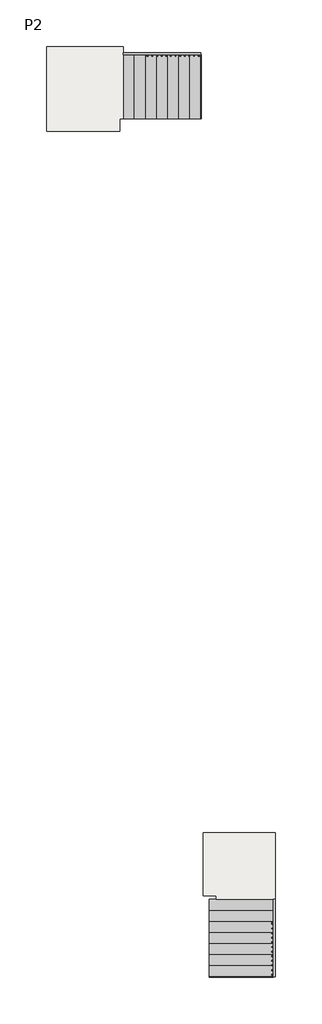
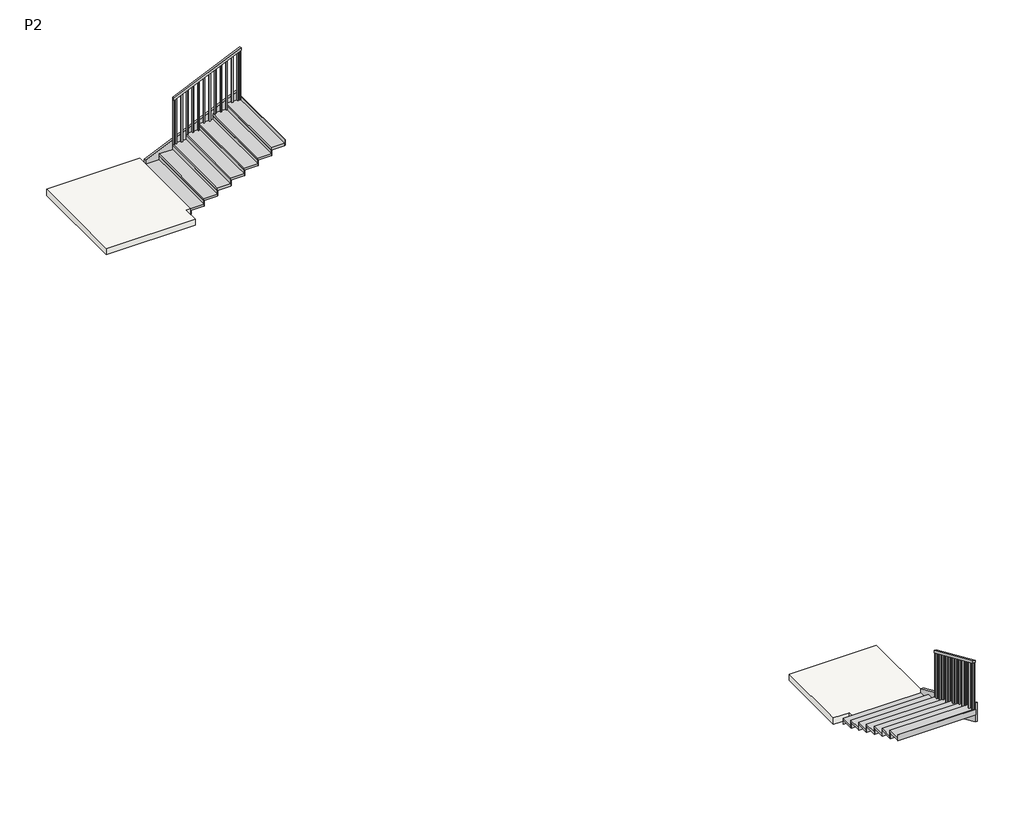
# One storey: 2 members, 2 railings, 2 slabs, 2 stair flights.
"""IFC4 building model written with IfcOpenShell, lengths in millimetres."""

import ifcopenshell
import ifcopenshell.guid

model = None  # the IFC model being written
_history = None  # IfcOwnerHistory: only IFC2X3 demands one
_inside = {}  # id of a spatial element -> (the spatial element, [elements in it])
_under = {}  # id of a project, library or spatial element -> (it, [spatial elements below it])
_declared = {}  # id of a project -> (the project, [libraries it declares])
_typed = {}  # id of a type object -> (the type object, [elements of that type])
_made_of = {}  # id of a material, layer set ... -> (it, [elements and type objects made of it])


def new_model(schema):
    """Start an empty IFC model of exactly this schema.

    Asked for "IFC4X3", IfcOpenShell would pick the latest addendum, in which some entities
    have other attributes; the version numbers below select the first issue.
    IFC2X3 requires an IfcOwnerHistory on every rooted entity: one is made here for all.
    """
    global model, _history
    if schema == "IFC4X3":
        model = ifcopenshell.file(schema_version=(4, 3, 0, 0))
    else:
        model = ifcopenshell.file(schema=schema)
    _inside.clear()
    _under.clear()
    _declared.clear()
    _typed.clear()
    _made_of.clear()
    _history = None
    if model.schema == "IFC2X3":
        org = make("IfcOrganization", Name="unknown")
        user = make(
            "IfcPersonAndOrganization",
            ThePerson=make("IfcPerson", FamilyName="unknown"),
            TheOrganization=org,
        )
        app = make(
            "IfcApplication",
            ApplicationDeveloper=org,
            Version="unknown",
            ApplicationFullName="unknown",
            ApplicationIdentifier="unknown",
        )
        _history = make(
            "IfcOwnerHistory",
            OwningUser=user,
            OwningApplication=app,
            ChangeAction="ADDED",
            CreationDate=0,
        )
    return model


def make(cls, **values):
    """One entity of the class cls with the attributes given. An attribute that is None is left unset."""
    return model.create_entity(
        cls, **{name: value for name, value in values.items() if value is not None}
    )


def rooted(cls, **values):
    """An entity with a GlobalId (a new one), such as an element, a storey or a relation."""
    return make(cls, GlobalId=ifcopenshell.guid.new(), OwnerHistory=_history, **values)


def si_unit(unit_type, name, prefix=None):
    """IfcSIUnit, for example si_unit("LENGTHUNIT", "METRE", prefix="MILLI")."""
    return make("IfcSIUnit", UnitType=unit_type, Prefix=prefix, Name=name)


def assignment(units):
    """IfcUnitAssignment: the units of a project."""
    return None if units is None else make("IfcUnitAssignment", Units=units)


def point(xyz):
    """IfcCartesianPoint."""
    return None if xyz is None else make("IfcCartesianPoint", Coordinates=xyz)


def direction(xyz):
    """IfcDirection."""
    return None if xyz is None else make("IfcDirection", DirectionRatios=xyz)


def frame(location, z_axis=None, x_axis=None):
    """IfcAxis2Placement3D, a coordinate frame: its origin and axes. An axis left out is left unset."""
    return make(
        "IfcAxis2Placement3D",
        Location=point(location),
        Axis=direction(z_axis),
        RefDirection=direction(x_axis),
    )


def origin():
    """The frame at (0, 0, 0) with its axes left unset."""
    return frame((0.0, 0.0, 0.0))


def place(relative_to, where):
    """IfcLocalPlacement: puts the frame where relative to a parent placement (None: the world)."""
    return make(
        "IfcLocalPlacement", PlacementRelTo=relative_to, RelativePlacement=where
    )


def context(
    kind, dimensions, precision=None, world=None, true_north=None, identifier=None
):
    """IfcGeometricRepresentationContext, for example the 3D "Model" context."""
    return make(
        "IfcGeometricRepresentationContext",
        ContextIdentifier=identifier,
        ContextType=kind,
        CoordinateSpaceDimension=dimensions,
        Precision=precision,
        WorldCoordinateSystem=world,
        TrueNorth=true_north,
    )


def project(units=None, contexts=None):
    """IfcProject with its units and contexts."""
    return rooted(
        "IfcProject",
        Name="project",
        RepresentationContexts=contexts,
        UnitsInContext=assignment(units),
    )


def spatial(cls, under=None, at=None, **own):
    """A site, building, storey or space (cls), placed at a placement, below another one or the project."""
    s = rooted(cls, ObjectPlacement=at, **own)
    if under is not None:
        _under.setdefault(under.id(), (under, []))[1].append(s)
    return s


def polyline(points):
    """IfcPolyline through the points."""
    return make("IfcPolyline", Points=[point(p) for p in points])


def outline(outer, holes=None, kind="AREA"):
    """IfcArbitraryClosedProfileDef: a profile drawn as a closed curve; with holes, ...WithVoids."""
    if holes is None:
        return make("IfcArbitraryClosedProfileDef", ProfileType=kind, OuterCurve=outer)
    return make(
        "IfcArbitraryProfileDefWithVoids",
        ProfileType=kind,
        OuterCurve=outer,
        InnerCurves=holes,
    )


def extrude(swept, where, along, depth):
    """IfcExtrudedAreaSolid: the profile swept, set in the frame where, extruded along a direction by depth."""
    return make(
        "IfcExtrudedAreaSolid",
        SweptArea=swept,
        Position=where,
        ExtrudedDirection=direction(along),
        Depth=depth,
    )


def shape(context_of_items, identifier, shape_type, items):
    """IfcShapeRepresentation: the items that make up one representation, for example the "Body"."""
    return make(
        "IfcShapeRepresentation",
        ContextOfItems=context_of_items,
        RepresentationIdentifier=identifier,
        RepresentationType=shape_type,
        Items=items,
    )


def source(mapping_origin, context_of_items, identifier, shape_type, items):
    """IfcRepresentationMap: a shape defined once, which mapped items show again and again."""
    return make(
        "IfcRepresentationMap",
        MappingOrigin=mapping_origin,
        MappedRepresentation=shape(context_of_items, identifier, shape_type, items),
    )


def transform(
    local_origin,
    x_axis=None,
    y_axis=None,
    z_axis=None,
    scale=None,
    scale2=None,
    scale3=None,
    uniform=True,
):
    """IfcCartesianTransformationOperator3D, or its non-uniform kind. x_axis, y_axis, z_axis: its Axis1, 2, 3."""
    if uniform:
        return make(
            "IfcCartesianTransformationOperator3D",
            Axis1=direction(x_axis),
            Axis2=direction(y_axis),
            LocalOrigin=point(local_origin),
            Scale=scale,
            Axis3=direction(z_axis),
        )
    return make(
        "IfcCartesianTransformationOperator3DnonUniform",
        Axis1=direction(x_axis),
        Axis2=direction(y_axis),
        LocalOrigin=point(local_origin),
        Scale=scale,
        Axis3=direction(z_axis),
        Scale2=scale2,
        Scale3=scale3,
    )


def mapped(mapping_source, mapping_target):
    """IfcMappedItem: shows the shape of a source again, moved by a transform."""
    return make(
        "IfcMappedItem", MappingSource=mapping_source, MappingTarget=mapping_target
    )


def made_of(thing, what):
    """Note that an element or type object is made of a material, layer set ...; save() writes the relation."""
    if what is not None:
        _made_of.setdefault(what.id(), (what, []))[1].append(thing)
    return thing


def element(
    cls,
    number,
    at=None,
    inside=None,
    cuts=None,
    type_object=None,
    material=None,
    context=None,
    identifier="Body",
    shape_type=None,
    held_by="IfcProductDefinitionShape",
    body=None,
    shapes=None,
    **own,
):
    """One element of the class cls, such as IfcWall. Its Tag is "e" and its number.

    at: its placement. inside: the storey or other place that contains it. cuts: it is an
    opening in that element (IfcRelVoidsElement). A single representation is given by context,
    identifier, shape_type and body (its items); several are given by shapes. held_by: the class
    of the entity that holds the representations. save() writes the other relations.
    """
    e = rooted(cls, Tag="e%d" % number, ObjectPlacement=at, **own)
    if body is not None:
        shapes = [shape(context, identifier, shape_type, body)]
    if shapes is not None:
        e.Representation = make(held_by, Representations=shapes)
    if inside is not None:
        _inside.setdefault(inside.id(), (inside, []))[1].append(e)
    if cuts is not None:
        rooted(
            "IfcRelVoidsElement", RelatingBuildingElement=cuts, RelatedOpeningElement=e
        )
    if type_object is not None:
        _typed.setdefault(type_object.id(), (type_object, []))[1].append(e)
    return made_of(e, material)


def aggregate(whole, parts):
    """IfcRelAggregates: a whole, such as a stair, and the parts it consists of."""
    return rooted("IfcRelAggregates", RelatingObject=whole, RelatedObjects=parts)


def save(model, path):
    """Write the relations noted so far, then the file.

    IfcRelAggregates (storeys below a building ...), IfcRelContainedInSpatialStructure (elements
    in a storey), IfcRelDefinesByType, IfcRelAssociatesMaterial and IfcRelDeclares: one each for
    every whole, place, type object, material and project.
    """
    for whole, parts in _under.values():
        aggregate(whole, parts)
    for where, things in _inside.values():
        rooted(
            "IfcRelContainedInSpatialStructure",
            RelatedElements=things,
            RelatingStructure=where,
        )
    for kind, things in _typed.values():
        rooted("IfcRelDefinesByType", RelatedObjects=things, RelatingType=kind)
    for what, things in _made_of.values():
        rooted("IfcRelAssociatesMaterial", RelatedObjects=things, RelatingMaterial=what)
    for by, libraries in _declared.values():
        rooted("IfcRelDeclares", RelatingContext=by, RelatedDefinitions=libraries)
    model.write(path)


def stair_flight_50mm_tread_13mm_riser_cadf6dc6(model_context):
    return source(origin(), model_context, "Body", "SweptSolid", [
        extrude(outline(polyline([(-15531.918089, 15530.6768963), (-15544.418089, 15530.6768963), (-15544.418089, 17260.6768963), (-15531.918089, 17260.6768963), (-15531.918089, 15530.6768963)])), frame((0.0, 0.0, -1066.6666667), z_axis=(0.0, 0.0, 1.0), x_axis=(1.0, 0.0, 0.0)), (0.0, 0.0, 1.0), 83.3333333),
        extrude(outline(polyline([(-15244.418089, 17260.6768963), (-15244.418089, 15530.6768963), (-15544.418089, 15530.6768963), (-15544.418089, 17260.6768963), (-15244.418089, 17260.6768963)])), frame((0.0, 0.0, -983.3333333), z_axis=(0.0, 0.0, 1.0), x_axis=(1.0, 0.0, 0.0)), (0.0, 0.0, 1.0), 50.0),
        extrude(outline(polyline([(-15231.918089, 15530.6768963), (-15244.418089, 15530.6768963), (-15244.418089, 17260.6768963), (-15231.918089, 17260.6768963), (-15231.918089, 15530.6768963)])), frame((0.0, 0.0, -983.3333333), z_axis=(0.0, 0.0, 1.0), x_axis=(1.0, 0.0, 0.0)), (0.0, 0.0, 1.0), 133.3333333),
        extrude(outline(polyline([(-14944.418089, 17260.6768963), (-14944.418089, 15530.6768963), (-15244.418089, 15530.6768963), (-15244.418089, 17260.6768963), (-14944.418089, 17260.6768963)])), frame((0.0, 0.0, -850.0), z_axis=(0.0, 0.0, 1.0), x_axis=(1.0, 0.0, 0.0)), (0.0, 0.0, 1.0), 50.0),
        extrude(outline(polyline([(-14931.918089, 15530.6768963), (-14944.418089, 15530.6768963), (-14944.418089, 17260.6768963), (-14931.918089, 17260.6768963), (-14931.918089, 15530.6768963)])), frame((0.0, 0.0, -850.0), z_axis=(0.0, 0.0, 1.0), x_axis=(1.0, 0.0, 0.0)), (0.0, 0.0, 1.0), 133.3333333),
        extrude(outline(polyline([(-14644.418089, 17260.6768963), (-14644.418089, 15530.6768963), (-14944.418089, 15530.6768963), (-14944.418089, 17260.6768963), (-14644.418089, 17260.6768963)])), frame((0.0, 0.0, -716.6666667), z_axis=(0.0, 0.0, 1.0), x_axis=(1.0, 0.0, 0.0)), (0.0, 0.0, 1.0), 50.0),
        extrude(outline(polyline([(-14631.918089, 15530.6768963), (-14644.418089, 15530.6768963), (-14644.418089, 17260.6768963), (-14631.918089, 17260.6768963), (-14631.918089, 15530.6768963)])), frame((0.0, 0.0, -716.6666667), z_axis=(0.0, 0.0, 1.0), x_axis=(1.0, 0.0, 0.0)), (0.0, 0.0, 1.0), 133.3333333),
        extrude(outline(polyline([(-14344.418089, 17260.6768963), (-14344.418089, 15530.6768963), (-14644.418089, 15530.6768963), (-14644.418089, 17260.6768963), (-14344.418089, 17260.6768963)])), frame((0.0, 0.0, -583.3333333), z_axis=(0.0, 0.0, 1.0), x_axis=(1.0, 0.0, 0.0)), (0.0, 0.0, 1.0), 50.0),
        extrude(outline(polyline([(-14331.918089, 15530.6768963), (-14344.418089, 15530.6768963), (-14344.418089, 17260.6768963), (-14331.918089, 17260.6768963), (-14331.918089, 15530.6768963)])), frame((0.0, 0.0, -583.3333333), z_axis=(0.0, 0.0, 1.0), x_axis=(1.0, 0.0, 0.0)), (0.0, 0.0, 1.0), 133.3333333),
        extrude(outline(polyline([(-14044.418089, 17260.6768963), (-14044.418089, 15530.6768963), (-14344.418089, 15530.6768963), (-14344.418089, 17260.6768963), (-14044.418089, 17260.6768963)])), frame((0.0, 0.0, -450.0), z_axis=(0.0, 0.0, 1.0), x_axis=(1.0, 0.0, 0.0)), (0.0, 0.0, 1.0), 50.0),
        extrude(outline(polyline([(-14031.918089, 15530.6768963), (-14044.418089, 15530.6768963), (-14044.418089, 17260.6768963), (-14031.918089, 17260.6768963), (-14031.918089, 15530.6768963)])), frame((0.0, 0.0, -450.0), z_axis=(0.0, 0.0, 1.0), x_axis=(1.0, 0.0, 0.0)), (0.0, 0.0, 1.0), 133.3333333),
        extrude(outline(polyline([(-13744.418089, 17260.6768963), (-13744.418089, 15530.6768963), (-14044.418089, 15530.6768963), (-14044.418089, 17260.6768963), (-13744.418089, 17260.6768963)])), frame((0.0, 0.0, -316.6666667), z_axis=(0.0, 0.0, 1.0), x_axis=(1.0, 0.0, 0.0)), (0.0, 0.0, 1.0), 50.0),
        extrude(outline(polyline([(-13731.918089, 15530.6768963), (-13744.418089, 15530.6768963), (-13744.418089, 17260.6768963), (-13731.918089, 17260.6768963), (-13731.918089, 15530.6768963)])), frame((0.0, 0.0, -316.6666667), z_axis=(0.0, 0.0, 1.0), x_axis=(1.0, 0.0, 0.0)), (0.0, 0.0, 1.0), 133.3333333),
        extrude(outline(polyline([(-13431.918089, 15530.6768963), (-13444.418089, 15530.6768963), (-13444.418089, 17260.6768963), (-13431.918089, 17260.6768963), (-13431.918089, 15530.6768963)])), frame((0.0, 0.0, -183.3333333), z_axis=(0.0, 0.0, 1.0), x_axis=(1.0, 0.0, 0.0)), (0.0, 0.0, 1.0), 133.3333333),
        extrude(outline(polyline([(-13444.418089, 17260.6768963), (-13444.418089, 15530.6768963), (-13744.418089, 15530.6768963), (-13744.418089, 17260.6768963), (-13444.418089, 17260.6768963)])), frame((0.0, 0.0, -183.3333333), z_axis=(0.0, 0.0, 1.0), x_axis=(1.0, 0.0, 0.0)), (0.0, 0.0, 1.0), 50.0),
    ])


def stair_flight_50mm_tread_13mm_riser_d40b31cd(model_context):
    return source(origin(), model_context, "Body", "SweptSolid", [
        extrude(outline(polyline([(-13215.2814495, -5630.5731037), (-13215.2814495, -5618.0731037), (-11485.2814495, -5618.0731037), (-11485.2814495, -5630.5731037), (-13215.2814495, -5630.5731037)])), frame((0.0, 0.0, -1066.6666667), z_axis=(0.0, 0.0, 1.0), x_axis=(1.0, 0.0, 0.0)), (0.0, 0.0, 1.0), 83.3333333),
        extrude(outline(polyline([(-11485.2814495, -5918.0731037), (-13215.2814495, -5918.0731037), (-13215.2814495, -5618.0731037), (-11485.2814495, -5618.0731037), (-11485.2814495, -5918.0731037)])), frame((0.0, 0.0, -983.3333333), z_axis=(0.0, 0.0, 1.0), x_axis=(1.0, 0.0, 0.0)), (0.0, 0.0, 1.0), 50.0),
        extrude(outline(polyline([(-13215.2814495, -5930.5731037), (-13215.2814495, -5918.0731037), (-11485.2814495, -5918.0731037), (-11485.2814495, -5930.5731037), (-13215.2814495, -5930.5731037)])), frame((0.0, 0.0, -983.3333333), z_axis=(0.0, 0.0, 1.0), x_axis=(1.0, 0.0, 0.0)), (0.0, 0.0, 1.0), 133.3333333),
        extrude(outline(polyline([(-11485.2814495, -6218.0731037), (-13215.2814495, -6218.0731037), (-13215.2814495, -5918.0731037), (-11485.2814495, -5918.0731037), (-11485.2814495, -6218.0731037)])), frame((0.0, 0.0, -850.0), z_axis=(0.0, 0.0, 1.0), x_axis=(1.0, 0.0, 0.0)), (0.0, 0.0, 1.0), 50.0),
        extrude(outline(polyline([(-13215.2814495, -6230.5731037), (-13215.2814495, -6218.0731037), (-11485.2814495, -6218.0731037), (-11485.2814495, -6230.5731037), (-13215.2814495, -6230.5731037)])), frame((0.0, 0.0, -850.0), z_axis=(0.0, 0.0, 1.0), x_axis=(1.0, 0.0, 0.0)), (0.0, 0.0, 1.0), 133.3333333),
        extrude(outline(polyline([(-11485.2814495, -6518.0731037), (-13215.2814495, -6518.0731037), (-13215.2814495, -6218.0731037), (-11485.2814495, -6218.0731037), (-11485.2814495, -6518.0731037)])), frame((0.0, 0.0, -716.6666667), z_axis=(0.0, 0.0, 1.0), x_axis=(1.0, 0.0, 0.0)), (0.0, 0.0, 1.0), 50.0),
        extrude(outline(polyline([(-13215.2814495, -6530.5731037), (-13215.2814495, -6518.0731037), (-11485.2814495, -6518.0731037), (-11485.2814495, -6530.5731037), (-13215.2814495, -6530.5731037)])), frame((0.0, 0.0, -716.6666667), z_axis=(0.0, 0.0, 1.0), x_axis=(1.0, 0.0, 0.0)), (0.0, 0.0, 1.0), 133.3333333),
        extrude(outline(polyline([(-11485.2814495, -6818.0731037), (-13215.2814495, -6818.0731037), (-13215.2814495, -6518.0731037), (-11485.2814495, -6518.0731037), (-11485.2814495, -6818.0731037)])), frame((0.0, 0.0, -583.3333333), z_axis=(0.0, 0.0, 1.0), x_axis=(1.0, 0.0, 0.0)), (0.0, 0.0, 1.0), 50.0),
        extrude(outline(polyline([(-13215.2814495, -6830.5731037), (-13215.2814495, -6818.0731037), (-11485.2814495, -6818.0731037), (-11485.2814495, -6830.5731037), (-13215.2814495, -6830.5731037)])), frame((0.0, 0.0, -583.3333333), z_axis=(0.0, 0.0, 1.0), x_axis=(1.0, 0.0, 0.0)), (0.0, 0.0, 1.0), 133.3333333),
        extrude(outline(polyline([(-11485.2814495, -7118.0731037), (-13215.2814495, -7118.0731037), (-13215.2814495, -6818.0731037), (-11485.2814495, -6818.0731037), (-11485.2814495, -7118.0731037)])), frame((0.0, 0.0, -450.0), z_axis=(0.0, 0.0, 1.0), x_axis=(1.0, 0.0, 0.0)), (0.0, 0.0, 1.0), 50.0),
        extrude(outline(polyline([(-13215.2814495, -7130.5731037), (-13215.2814495, -7118.0731037), (-11485.2814495, -7118.0731037), (-11485.2814495, -7130.5731037), (-13215.2814495, -7130.5731037)])), frame((0.0, 0.0, -450.0), z_axis=(0.0, 0.0, 1.0), x_axis=(1.0, 0.0, 0.0)), (0.0, 0.0, 1.0), 133.3333333),
        extrude(outline(polyline([(-11485.2814495, -7418.0731037), (-13215.2814495, -7418.0731037), (-13215.2814495, -7118.0731037), (-11485.2814495, -7118.0731037), (-11485.2814495, -7418.0731037)])), frame((0.0, 0.0, -316.6666667), z_axis=(0.0, 0.0, 1.0), x_axis=(1.0, 0.0, 0.0)), (0.0, 0.0, 1.0), 50.0),
        extrude(outline(polyline([(-13215.2814495, -7430.5731037), (-13215.2814495, -7418.0731037), (-11485.2814495, -7418.0731037), (-11485.2814495, -7430.5731037), (-13215.2814495, -7430.5731037)])), frame((0.0, 0.0, -316.6666667), z_axis=(0.0, 0.0, 1.0), x_axis=(1.0, 0.0, 0.0)), (0.0, 0.0, 1.0), 133.3333333),
        extrude(outline(polyline([(-13215.2814495, -7730.5731037), (-13215.2814495, -7718.0731037), (-11485.2814495, -7718.0731037), (-11485.2814495, -7730.5731037), (-13215.2814495, -7730.5731037)])), frame((0.0, 0.0, -183.3333333), z_axis=(0.0, 0.0, 1.0), x_axis=(1.0, 0.0, 0.0)), (0.0, 0.0, 1.0), 133.3333333),
        extrude(outline(polyline([(-11485.2814495, -7718.0731037), (-13215.2814495, -7718.0731037), (-13215.2814495, -7418.0731037), (-11485.2814495, -7418.0731037), (-11485.2814495, -7718.0731037)])), frame((0.0, 0.0, -183.3333333), z_axis=(0.0, 0.0, 1.0), x_axis=(1.0, 0.0, 0.0)), (0.0, 0.0, 1.0), 50.0),
    ])


model = new_model("IFC4")

# Units and contexts
model_context = context("Model", 3, world=origin())
ifc_project = project(units=[si_unit("LENGTHUNIT", "METRE", prefix="MILLI")], contexts=[model_context])

# Site, building, storey
site = spatial("IfcSite", under=ifc_project)
building = spatial("IfcBuilding", under=site)
storey = spatial("IfcBuildingStorey", under=building, Name="P2", Elevation=-1066.6666667)

# Members
placement = place(None, origin())
element("IfcMember", 1, ObjectType="Stringer - 50mm Width", at=placement, inside=storey, context=model_context, shape_type="SweptSolid", body=[
    extrude(outline(polyline([(-848.6428388, -15544.418089), (-1066.6666667, -15544.418089), (-1066.6666667, -15050.0859214), (-353.0365189, -13444.418089), (84.6904945, -13444.418089), (-848.6428388, -15544.418089)])), frame((0.0, 17260.6768963, 0.0), z_axis=(0.0, 1.0, 0.0), x_axis=(0.0, 0.0, 1.0)), (0.0, 0.0, 1.0), 50.0),
])
element("IfcMember", 2, ObjectType="Stringer - 50mm Width", at=placement, inside=storey, context=model_context, shape_type="SweptSolid", body=[
    extrude(outline(polyline([(-5618.0731037, -848.6428388), (-5618.0731037, -1066.6666667), (-6112.4052712, -1066.6666667), (-7718.0731037, -353.0365189), (-7718.0731037, 84.6904945), (-5618.0731037, -848.6428388)])), frame((-11485.2814495, 0.0, 0.0), z_axis=(1.0, 0.0, 0.0), x_axis=(0.0, 1.0, 0.0)), (0.0, 0.0, 1.0), 50.0),
])

# Railings
element("IfcRailing", 3, ObjectType="1100mm", at=placement, inside=storey, context=model_context, shape_type="SweptSolid", body=[
    extrude(outline(polyline([(433.3333333, -14944.418089), (378.6174567, -14944.418089), (1045.2841233, -13444.418089), (1100.0, -13444.418089), (433.3333333, -14944.418089)])), frame((0.0, 17210.2768963, 0.0), z_axis=(0.0, 1.0, 0.0), x_axis=(0.0, 0.0, 1.0)), (0.0, 0.0, 1.0), 50.0),
    extrude(outline(polyline([(-133.3333333, -13519.418089), (-133.3333333, -13494.418089), (1023.0619011, -13494.418089), (1011.95079, -13519.418089), (-133.3333333, -13519.418089)])), frame((0.0, 17222.7768963, 0.0), z_axis=(0.0, 1.0, 0.0), x_axis=(0.0, 0.0, 1.0)), (0.0, 0.0, 1.0), 25.0),
    extrude(outline(polyline([(-133.3333333, -13644.418089), (-133.3333333, -13619.418089), (967.5063455, -13619.418089), (956.3952344, -13644.418089), (-133.3333333, -13644.418089)])), frame((0.0, 17222.7768963, 0.0), z_axis=(0.0, 1.0, 0.0), x_axis=(0.0, 0.0, 1.0)), (0.0, 0.0, 1.0), 25.0),
    extrude(outline(polyline([(-266.6666667, -13769.418089), (-266.6666667, -13744.418089), (911.95079, -13744.418089), (900.8396789, -13769.418089), (-266.6666667, -13769.418089)])), frame((0.0, 17222.7768963, 0.0), z_axis=(0.0, 1.0, 0.0), x_axis=(0.0, 0.0, 1.0)), (0.0, 0.0, 1.0), 25.0),
    extrude(outline(polyline([(-266.6666667, -13894.418089), (-266.6666667, -13869.418089), (856.3952344, -13869.418089), (845.2841233, -13894.418089), (-266.6666667, -13894.418089)])), frame((0.0, 17222.7768963, 0.0), z_axis=(0.0, 1.0, 0.0), x_axis=(0.0, 0.0, 1.0)), (0.0, 0.0, 1.0), 25.0),
    extrude(outline(polyline([(-266.6666667, -14019.418089), (-266.6666667, -13994.418089), (800.8396789, -13994.418089), (789.7285678, -14019.418089), (-266.6666667, -14019.418089)])), frame((0.0, 17222.7768963, 0.0), z_axis=(0.0, 1.0, 0.0), x_axis=(0.0, 0.0, 1.0)), (0.0, 0.0, 1.0), 25.0),
    extrude(outline(polyline([(-400.0, -14144.418089), (-400.0, -14119.418089), (745.2841233, -14119.418089), (734.1730122, -14144.418089), (-400.0, -14144.418089)])), frame((0.0, 17222.7768963, 0.0), z_axis=(0.0, 1.0, 0.0), x_axis=(0.0, 0.0, 1.0)), (0.0, 0.0, 1.0), 25.0),
    extrude(outline(polyline([(-400.0, -14269.418089), (-400.0, -14244.418089), (689.7285678, -14244.418089), (678.6174567, -14269.418089), (-400.0, -14269.418089)])), frame((0.0, 17222.7768963, 0.0), z_axis=(0.0, 1.0, 0.0), x_axis=(0.0, 0.0, 1.0)), (0.0, 0.0, 1.0), 25.0),
    extrude(outline(polyline([(-533.3333333, -14394.418089), (-533.3333333, -14369.418089), (634.1730122, -14369.418089), (623.0619011, -14394.418089), (-533.3333333, -14394.418089)])), frame((0.0, 17222.7768963, 0.0), z_axis=(0.0, 1.0, 0.0), x_axis=(0.0, 0.0, 1.0)), (0.0, 0.0, 1.0), 25.0),
    extrude(outline(polyline([(-533.3333333, -14519.418089), (-533.3333333, -14494.418089), (578.6174567, -14494.418089), (567.5063455, -14519.418089), (-533.3333333, -14519.418089)])), frame((0.0, 17222.7768963, 0.0), z_axis=(0.0, 1.0, 0.0), x_axis=(0.0, 0.0, 1.0)), (0.0, 0.0, 1.0), 25.0),
    extrude(outline(polyline([(-533.3333333, -14644.418089), (-533.3333333, -14619.418089), (523.0619011, -14619.418089), (511.95079, -14644.418089), (-533.3333333, -14644.418089)])), frame((0.0, 17222.7768963, 0.0), z_axis=(0.0, 1.0, 0.0), x_axis=(0.0, 0.0, 1.0)), (0.0, 0.0, 1.0), 25.0),
    extrude(outline(polyline([(-666.6666667, -14769.418089), (-666.6666667, -14744.418089), (467.5063455, -14744.418089), (456.3952344, -14769.418089), (-666.6666667, -14769.418089)])), frame((0.0, 17222.7768963, 0.0), z_axis=(0.0, 1.0, 0.0), x_axis=(0.0, 0.0, 1.0)), (0.0, 0.0, 1.0), 25.0),
    extrude(outline(polyline([(-666.6666667, -14894.418089), (-666.6666667, -14869.418089), (411.95079, -14869.418089), (400.8396789, -14894.418089), (-666.6666667, -14894.418089)])), frame((0.0, 17222.7768963, 0.0), z_axis=(0.0, 1.0, 0.0), x_axis=(0.0, 0.0, 1.0)), (0.0, 0.0, 1.0), 25.0),
    extrude(outline(polyline([(-133.3333333, -13469.418089), (-133.3333333, -13444.418089), (1045.2841233, -13444.418089), (1034.1730122, -13469.418089), (-133.3333333, -13469.418089)])), frame((0.0, 17222.7768963, 0.0), z_axis=(0.0, 1.0, 0.0), x_axis=(0.0, 0.0, 1.0)), (0.0, 0.0, 1.0), 25.0),
    extrude(outline(polyline([(-666.6666667, -14944.418089), (-666.6666667, -14919.418089), (389.7285678, -14919.418089), (378.6174567, -14944.418089), (-666.6666667, -14944.418089)])), frame((0.0, 17222.7768963, 0.0), z_axis=(0.0, 1.0, 0.0), x_axis=(0.0, 0.0, 1.0)), (0.0, 0.0, 1.0), 25.0),
])
element("IfcRailing", 4, ObjectType="1100mm", at=placement, inside=storey, context=model_context, shape_type="SweptSolid", body=[
    extrude(outline(polyline([(-6218.0731037, 433.3333333), (-6218.0731037, 378.6174567), (-7718.0731037, 1045.2841233), (-7718.0731037, 1100.0), (-6218.0731037, 433.3333333)])), frame((-11535.6814495, 0.0, 0.0), z_axis=(1.0, 0.0, 0.0), x_axis=(0.0, 1.0, 0.0)), (0.0, 0.0, 1.0), 50.0),
    extrude(outline(polyline([(-7643.0731037, -133.3333333), (-7668.0731037, -133.3333333), (-7668.0731037, 1023.0619011), (-7643.0731037, 1011.95079), (-7643.0731037, -133.3333333)])), frame((-11523.1814495, 0.0, 0.0), z_axis=(1.0, 0.0, 0.0), x_axis=(0.0, 1.0, 0.0)), (0.0, 0.0, 1.0), 25.0),
    extrude(outline(polyline([(-7518.0731037, -133.3333333), (-7543.0731037, -133.3333333), (-7543.0731037, 967.5063455), (-7518.0731037, 956.3952344), (-7518.0731037, -133.3333333)])), frame((-11523.1814495, 0.0, 0.0), z_axis=(1.0, 0.0, 0.0), x_axis=(0.0, 1.0, 0.0)), (0.0, 0.0, 1.0), 25.0),
    extrude(outline(polyline([(-7393.0731037, -266.6666667), (-7418.0731037, -266.6666667), (-7418.0731037, 911.95079), (-7393.0731037, 900.8396789), (-7393.0731037, -266.6666667)])), frame((-11523.1814495, 0.0, 0.0), z_axis=(1.0, 0.0, 0.0), x_axis=(0.0, 1.0, 0.0)), (0.0, 0.0, 1.0), 25.0),
    extrude(outline(polyline([(-7268.0731037, -266.6666667), (-7293.0731037, -266.6666667), (-7293.0731037, 856.3952344), (-7268.0731037, 845.2841233), (-7268.0731037, -266.6666667)])), frame((-11523.1814495, 0.0, 0.0), z_axis=(1.0, 0.0, 0.0), x_axis=(0.0, 1.0, 0.0)), (0.0, 0.0, 1.0), 25.0),
    extrude(outline(polyline([(-7143.0731037, -266.6666667), (-7168.0731037, -266.6666667), (-7168.0731037, 800.8396789), (-7143.0731037, 789.7285678), (-7143.0731037, -266.6666667)])), frame((-11523.1814495, 0.0, 0.0), z_axis=(1.0, 0.0, 0.0), x_axis=(0.0, 1.0, 0.0)), (0.0, 0.0, 1.0), 25.0),
    extrude(outline(polyline([(-7018.0731037, -400.0), (-7043.0731037, -400.0), (-7043.0731037, 745.2841233), (-7018.0731037, 734.1730122), (-7018.0731037, -400.0)])), frame((-11523.1814495, 0.0, 0.0), z_axis=(1.0, 0.0, 0.0), x_axis=(0.0, 1.0, 0.0)), (0.0, 0.0, 1.0), 25.0),
    extrude(outline(polyline([(-6893.0731037, -400.0), (-6918.0731037, -400.0), (-6918.0731037, 689.7285678), (-6893.0731037, 678.6174567), (-6893.0731037, -400.0)])), frame((-11523.1814495, 0.0, 0.0), z_axis=(1.0, 0.0, 0.0), x_axis=(0.0, 1.0, 0.0)), (0.0, 0.0, 1.0), 25.0),
    extrude(outline(polyline([(-6768.0731037, -533.3333333), (-6793.0731037, -533.3333333), (-6793.0731037, 634.1730122), (-6768.0731037, 623.0619011), (-6768.0731037, -533.3333333)])), frame((-11523.1814495, 0.0, 0.0), z_axis=(1.0, 0.0, 0.0), x_axis=(0.0, 1.0, 0.0)), (0.0, 0.0, 1.0), 25.0),
    extrude(outline(polyline([(-6643.0731037, -533.3333333), (-6668.0731037, -533.3333333), (-6668.0731037, 578.6174567), (-6643.0731037, 567.5063455), (-6643.0731037, -533.3333333)])), frame((-11523.1814495, 0.0, 0.0), z_axis=(1.0, 0.0, 0.0), x_axis=(0.0, 1.0, 0.0)), (0.0, 0.0, 1.0), 25.0),
    extrude(outline(polyline([(-6518.0731037, -533.3333333), (-6543.0731037, -533.3333333), (-6543.0731037, 523.0619011), (-6518.0731037, 511.95079), (-6518.0731037, -533.3333333)])), frame((-11523.1814495, 0.0, 0.0), z_axis=(1.0, 0.0, 0.0), x_axis=(0.0, 1.0, 0.0)), (0.0, 0.0, 1.0), 25.0),
    extrude(outline(polyline([(-6393.0731037, -666.6666667), (-6418.0731037, -666.6666667), (-6418.0731037, 467.5063455), (-6393.0731037, 456.3952344), (-6393.0731037, -666.6666667)])), frame((-11523.1814495, 0.0, 0.0), z_axis=(1.0, 0.0, 0.0), x_axis=(0.0, 1.0, 0.0)), (0.0, 0.0, 1.0), 25.0),
    extrude(outline(polyline([(-6268.0731037, -666.6666667), (-6293.0731037, -666.6666667), (-6293.0731037, 411.95079), (-6268.0731037, 400.8396789), (-6268.0731037, -666.6666667)])), frame((-11523.1814495, 0.0, 0.0), z_axis=(1.0, 0.0, 0.0), x_axis=(0.0, 1.0, 0.0)), (0.0, 0.0, 1.0), 25.0),
    extrude(outline(polyline([(-7693.0731037, -133.3333333), (-7718.0731037, -133.3333333), (-7718.0731037, 1045.2841233), (-7693.0731037, 1034.1730122), (-7693.0731037, -133.3333333)])), frame((-11523.1814495, 0.0, 0.0), z_axis=(1.0, 0.0, 0.0), x_axis=(0.0, 1.0, 0.0)), (0.0, 0.0, 1.0), 25.0),
    extrude(outline(polyline([(-6218.0731037, -666.6666667), (-6243.0731037, -666.6666667), (-6243.0731037, 389.7285678), (-6218.0731037, 378.6174567), (-6218.0731037, -666.6666667)])), frame((-11523.1814495, 0.0, 0.0), z_axis=(1.0, 0.0, 0.0), x_axis=(0.0, 1.0, 0.0)), (0.0, 0.0, 1.0), 25.0),
])

# Slabs
element("IfcSlab", 5, ObjectType="Generic 150mm", at=placement, inside=storey, context=model_context, shape_type="SweptSolid", body=[
    extrude(outline(polyline([(-15544.418089, 15530.6768963), (-15644.418089, 15530.6768963), (-15644.418089, 15180.6768963), (-17624.418089, 15180.6768963), (-17624.418089, 17480.6768963), (-15544.418089, 17480.6768963), (-15544.418089, 15530.6768963)])), frame((0.0, 0.0, -1083.3333333), z_axis=(0.0, 0.0, 1.0), x_axis=(1.0, 0.0, 0.0)), (0.0, 0.0, 1.0), 150.0),
])
element("IfcSlab", 6, ObjectType="Generic 150mm", at=placement, inside=storey, context=model_context, shape_type="SweptSolid", body=[
    extrude(outline(polyline([(-13025.2814495, -5618.0731037), (-13025.2814495, -5518.0731037), (-13375.2814495, -5518.0731037), (-13375.2814495, -3818.0731037), (-11434.418089, -3818.0731037), (-11434.418089, -5618.0731037), (-13025.2814495, -5618.0731037)])), frame((0.0, 0.0, -1083.3333333), z_axis=(0.0, 0.0, 1.0), x_axis=(1.0, 0.0, 0.0)), (0.0, 0.0, 1.0), 150.0),
])

# Stair flights
stair_flight_50mm_tread_13mm_riser_shape = stair_flight_50mm_tread_13mm_riser_cadf6dc6(model_context)
element("IfcStairFlight", 7, ObjectType="50mm Tread 13mm Riser", at=placement, inside=storey, context=model_context, shape_type="MappedRepresentation", body=[
    mapped(stair_flight_50mm_tread_13mm_riser_shape, transform((0.0, 0.0, 0.0), x_axis=(1.0, 0.0, 0.0), y_axis=(0.0, 1.0, 0.0), z_axis=(0.0, 0.0, 1.0))),
])
stair_flight_50mm_tread_13mm_riser_2_shape = stair_flight_50mm_tread_13mm_riser_d40b31cd(model_context)
element("IfcStairFlight", 8, ObjectType="50mm Tread 13mm Riser", at=placement, inside=storey, context=model_context, shape_type="MappedRepresentation", body=[
    mapped(stair_flight_50mm_tread_13mm_riser_2_shape, transform((0.0, 0.0, 0.0), x_axis=(1.0, 0.0, 0.0), y_axis=(0.0, 1.0, 0.0), z_axis=(0.0, 0.0, 1.0))),
])

save(model, "model.ifc")

# Revit data of these elements
# Type "1100mm"
#   built-in parameter 1008612 = 0.019685 (stored number, unit not read)
#   built-in parameter 1008611 = 0.019685 (stored number, unit not read)
#   built-in parameter 1008609 = 0.902231 (stored number, unit not read)
#   built-in parameter 1008604 = 0.19685 (stored number, unit not read)
#   built-in parameter 1008603 = 0.164042 (stored number, unit not read)
#   Railing Height = 110 cm
#   built-in parameter 1008630 = 2
#   built-in parameter 1008610 = 2
#   built-in parameter 1008608 = 1
#   built-in parameter 1008618 = M_Baluster - Square : 25mm
# Type "Generic 150mm"
#   Function = 0
#   Layers, outside or top first: 15 cm no material (function 1)
# Elements 1, 2 (IfcMember, "Stringer - 50mm Width")
#   Phase Created = New Construction
# Elements 3, 4 (IfcRailing, "1100mm")
#   Phase Created = New Construction
# Element 5 (IfcSlab, "Generic 150mm")
#   built-in parameter 1001955 = -1.5708 (stored number, unit not read)
#   Height Offset From Level = 13.3333 cm
#   Phase Created = New Construction
#   Materials on its faces: "Default Floor"
# Element 6 (IfcSlab, "Generic 150mm")
#   built-in parameter 1001955 = 3.14159 (stored number, unit not read)
#   Height Offset From Level = 13.3333 cm
#   Phase Created = New Construction
#   Materials on its faces: "Default Floor"
# Elements 7, 8 (IfcStairFlight, "50mm Tread 13mm Riser")
#   Phase Created = New Construction
# Materials
#   "Default Floor": class "Miscellaneous", colour RGB 127 127 127, transparency 0, Cost = 0
